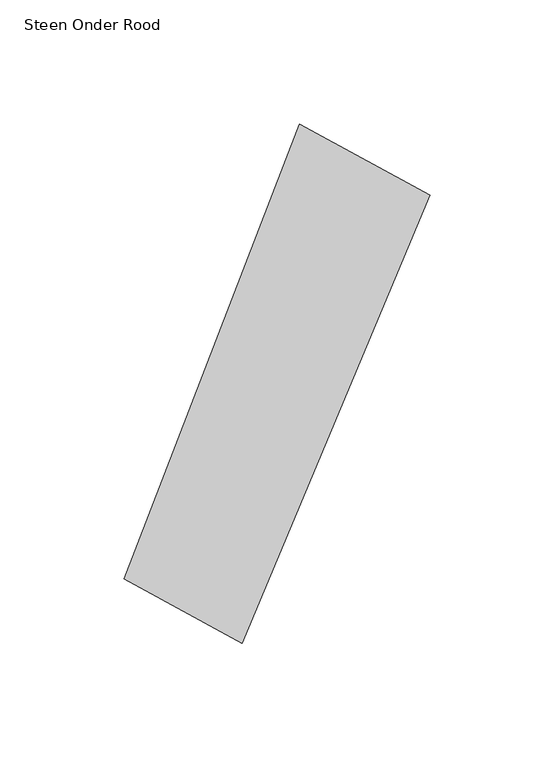
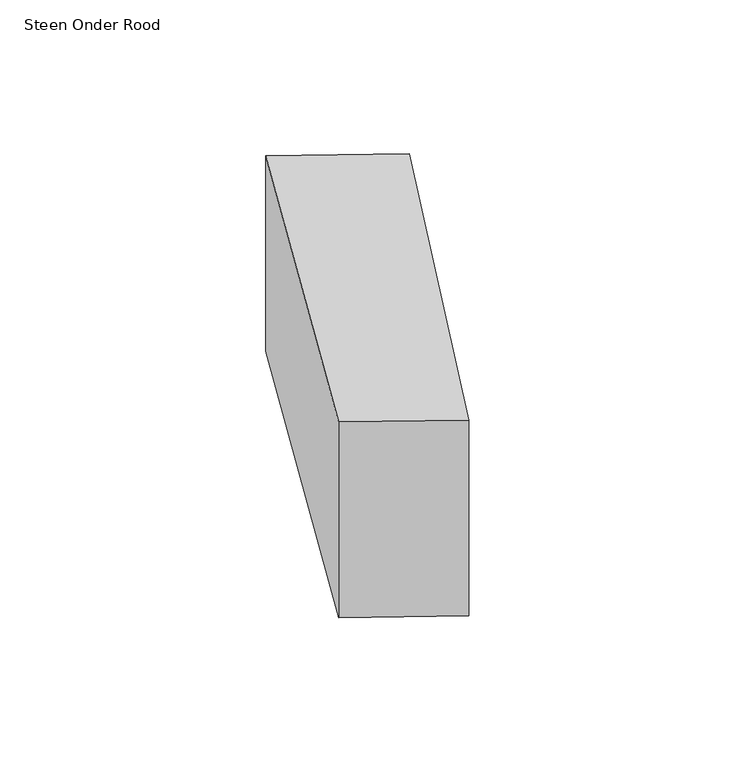
"""IFC4 building model written with IfcOpenShell, lengths in millimetres: proxy geometry, 00_GMA_steen_versie_4 : Steen Onder Rood."""

from ifc_helpers import new_model, si_unit, origin, origin_with_axes, place, context, project, spatial, polyline, outline, extrude, source, transform, mapped, element, save


def steen_onder_rood_3e976bb6(model_context):
    return source(origin(), model_context, "Body", "SweptSolid", [
        extrude(outline(polyline([(138.081587, 159.0882561), (62.3111083, -21.7225173), (14.6199118, 4.2558434), (85.3891047, 187.8072572), (138.081587, 159.0882561)])), origin_with_axes(), (0.0, 0.0, 1.0), 100.0),
    ])


if __name__ == "__main__":
    model = new_model("IFC4")
    model_context = context("Model", 3, world=origin())
    ifc_project = project(units=[si_unit("LENGTHUNIT", "METRE", prefix="MILLI")], contexts=[model_context])
    site = spatial("IfcSite", under=ifc_project)
    building = spatial("IfcBuilding", under=site)
    placement = place(None, origin())
    steen_onder_rood_shape = steen_onder_rood_3e976bb6(model_context)
    element("IfcBuildingElementProxy", 1, Name="00_GMA_steen_versie_4 : Steen Onder Rood", ObjectType="00_GMA_steen_versie_4 : Steen Onder Rood", at=placement, inside=building, context=model_context, shape_type="MappedRepresentation", body=[
        mapped(steen_onder_rood_shape, transform((0.0, 0.0, 0.0), x_axis=(1.0, 0.0, 0.0), y_axis=(0.0, 1.0, 0.0), z_axis=(0.0, 0.0, 1.0))),
    ])
    save(model, "model.ifc")

# Revit data of these elements
# Type "00_GMA_steen_versie_4 : Steen Onder Rood"
#   StootVoegHalfBoven [instance default] = 5 mm
#   StootVoegHalf [instance default] = 5 mm
#   StootVoegBreedteOnder = 10 mm
#   StootVoegBreedteBoven = 10 mm
#   Steendikte = 100 mm
#   LintVoegOnderHalf = 0 mm
#   LintVoegOnder = 0 mm
#   LintVoegBovenHalf = 5 mm
#   LintVoegBoven = 10 mm
#   materiaal = 21_steen_rood
#   MateriaalVoeg = none
#   Default Elevation = 0
# Element 1 (IfcBuildingElementProxy, "00_GMA_steen_versie_4 : Steen Onder Rood")
#   Materials on its faces: "21_steen_rood"
# Materials
#   "21_steen_rood": class "Unassigned", colour RGB 213 111 43, transparency 0, Cost = 0
